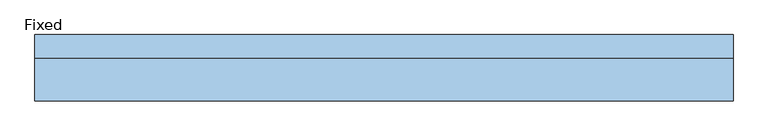
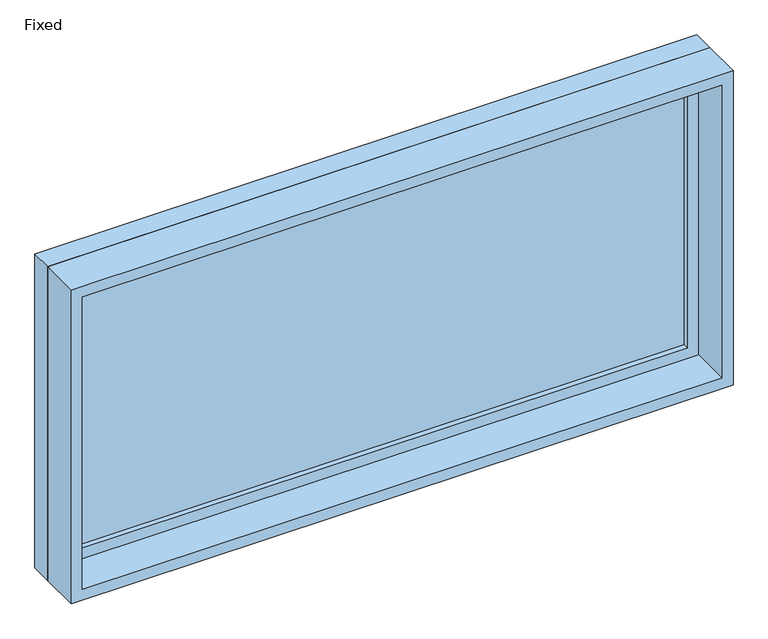
"""IFC4 building model written with IfcOpenShell, lengths in millimetres: window geometry, Fixed."""

from ifc_helpers import new_model, si_unit, frame, origin, place, context, project, spatial, polyline, outline, extrude, source, transform, mapped, element, save


def fixed_39c3167b(model_context):
    return source(origin(), model_context, "Body", "SweptSolid", [
        extrude(outline(polyline([(835.025, 41.275), (-911.225, 41.275), (-911.225, 53.975), (835.025, 53.975), (835.025, 41.275)])), frame((0.0, 0.0, 1257.3), z_axis=(0.0, 0.0, 1.0), x_axis=(1.0, 0.0, 0.0)), (0.0, 0.0, 1.0), 812.8),
        extrude(outline(polyline([(2114.55, -955.675), (1212.85, -955.675), (1212.85, 879.475), (2114.55, 879.475), (2114.55, -955.675)]), holes=[polyline([(2070.1, -911.225), (2070.1, 835.025), (1257.3, 835.025), (1257.3, -911.225), (2070.1, -911.225)])]), frame((0.0, 25.4, 0.0), z_axis=(0.0, 1.0, 0.0), x_axis=(0.0, 0.0, 1.0)), (0.0, 0.0, 1.0), 44.45),
        extrude(outline(polyline([(2133.6, -974.725), (1193.8, -974.725), (1193.8, 898.525), (2133.6, 898.525), (2133.6, -974.725)]), holes=[polyline([(2101.85, -942.975), (2101.85, 866.775), (1225.55, 866.775), (1225.55, -942.975), (2101.85, -942.975)])]), frame((0.0, -88.9, 0.0), z_axis=(0.0, 1.0, 0.0), x_axis=(0.0, 0.0, 1.0)), (0.0, 0.0, 1.0), 114.3),
        extrude(outline(polyline([(2133.6, 898.525), (2133.6, -974.725), (1193.8, -974.725), (1193.8, 898.525), (2133.6, 898.525)]), holes=[polyline([(2114.55, 879.475), (1212.85, 879.475), (1212.85, -955.675), (2114.55, -955.675), (2114.55, 879.475)])]), frame((0.0, 25.4, 0.0), z_axis=(0.0, 1.0, 0.0), x_axis=(0.0, 0.0, 1.0)), (0.0, 0.0, 1.0), 63.5),
    ])


if __name__ == "__main__":
    model = new_model("IFC4")
    model_context = context("Model", 3, world=origin())
    ifc_project = project(units=[si_unit("LENGTHUNIT", "METRE", prefix="MILLI")], contexts=[model_context])
    site = spatial("IfcSite", under=ifc_project)
    building = spatial("IfcBuilding", under=site)
    placement = place(None, origin())
    fixed_shape = fixed_39c3167b(model_context)
    element("IfcWindow", 1, ObjectType="Fixed : 6' 1 34\"\" x 3' 1\"", at=placement, inside=building, context=model_context, shape_type="MappedRepresentation", body=[
        mapped(fixed_shape, transform((0.0, 0.0, 0.0), x_axis=(1.0, 0.0, 0.0), y_axis=(0.0, 1.0, 0.0), z_axis=(0.0, 0.0, 1.0))),
    ])
    save(model, "model.ifc")

# Revit data of these elements
# Type "Fixed : 6' 1 34\"\" x 3' 1\""
#   Type Mark = "10"
#   Assembly Code = "B2020100"
#   Height = 3' - 1"
#   Default Sill Height = 3' - 11"
#   Width = 6' - 1 3/4"
#   Window Inset = 0' - 0 3/4"
#   Glass Pane Material = Glass
#   Sash Material = Sash
#   Wall Closure = (empty or 0)
# Element 1 (IfcWindow, "Fixed : 6' 1 34\"\" x 3' 1\"")
#   Materials on its faces: "Sash", "Glass"
# Materials
#   "Glass": class "Glass", colour RGB 218 227 224, transparency 0.85, Description = "Soda Lime Glass", Cost = 0
#   "Sash": class "Wood", colour RGB 136 99 55, transparency 0
